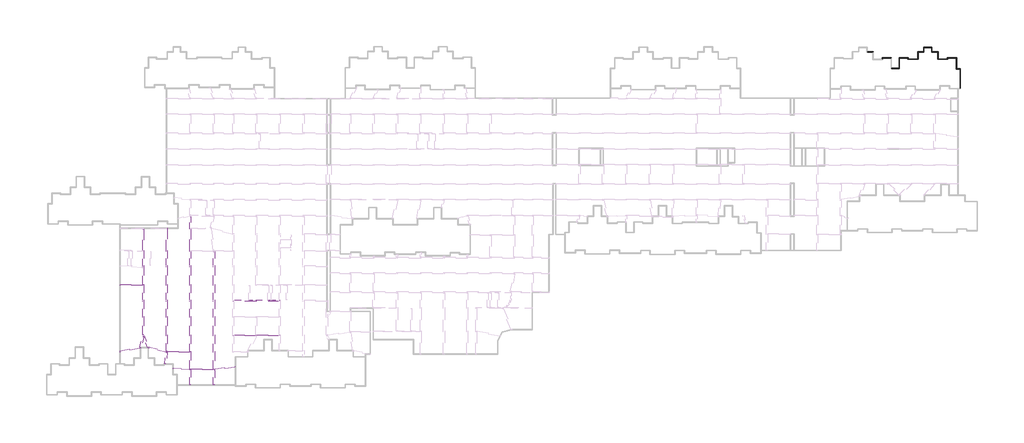
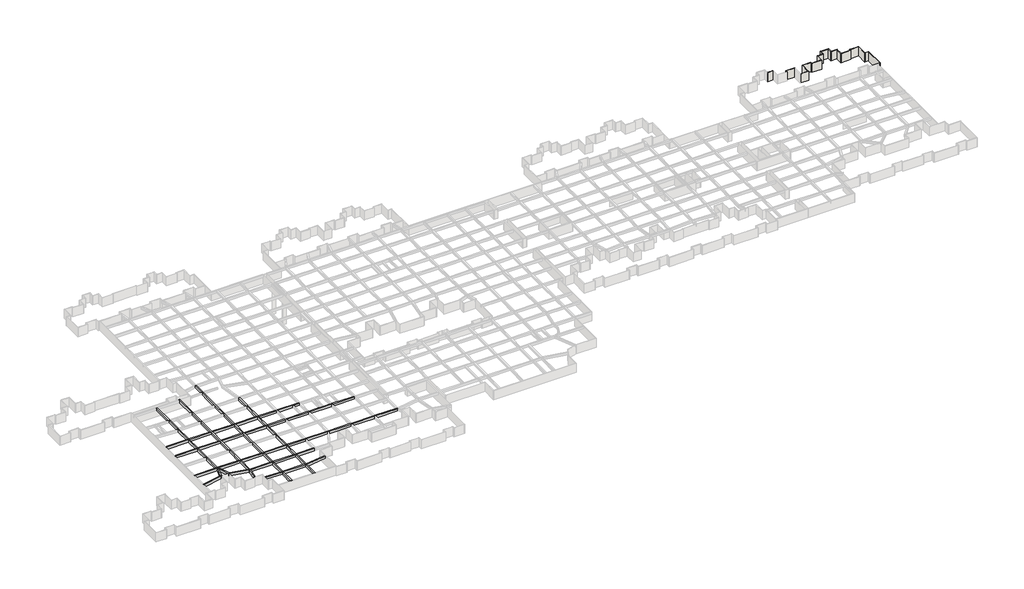
# One storey, part 9 of 16: 21 walls, 16 beams.
"""IFC4 building model written with IfcOpenShell, lengths in millimetres."""

from ifc_helpers import new_model, si_unit, frame, origin, place, context, project, spatial, polyline, outline, extrude, faceted_brep, element, save

model = new_model("IFC4")

# Units and contexts
model_context = context("Model", 3, world=origin())
ifc_project = project(units=[si_unit("LENGTHUNIT", "METRE", prefix="MILLI")], contexts=[model_context])

# Site, building, storey
site = spatial("IfcSite", under=ifc_project)
building = spatial("IfcBuilding", under=site)
storey = spatial("IfcBuildingStorey", under=building, Name="户型图", Elevation=0.0)

# Beams
placement = place(None, origin())
element("IfcBeam", 1, ObjectType="混凝土 - 矩形梁 : KL_beam", at=placement, inside=storey, context=model_context, shape_type="Brep", body=[
    faceted_brep([(208521.0257524, -230392.9293423, 3300.0), (208121.0257524, -230392.9293423, 3300.0), (208121.0257524, -230392.9293423, 2500.0), (208521.0257524, -230392.9293423, 2500.0), (208521.0257524, -225207.0649746, 3300.0), (208521.0257524, -224807.0649746, 3300.0), (208521.0257524, -219234.8916503, 3300.0), (208521.0257524, -218834.8916503, 3300.0), (208521.0257524, -213630.8034485, 3300.0), (208521.0257524, -213230.8034485, 3300.0), (208521.0257524, -207265.1471774, 3300.0), (208521.0257524, -206865.1471774, 3300.0), (208521.0257524, -201765.1471774, 3300.0), (208521.0257524, -201365.1471774, 3300.0), (208521.0257524, -196365.1471774, 3300.0), (208521.0257524, -195965.1471774, 3300.0), (208521.0257524, -189965.1471774, 3300.0), (208521.0257524, -189565.1471774, 3300.0), (208521.0257524, -184765.1471774, 3300.0), (208521.0257524, -184365.1471774, 3300.0), (208521.0257524, -177055.1471774, 3300.0), (208521.0257524, -176755.1471774, 3300.0), (208521.0257524, -172734.8916503, 3300.0), (208320.403704, -172734.8916503, 3300.0), (208121.0257524, -172780.9216773, 3300.0), (208121.0257524, -176755.1471774, 3300.0), (208121.0257524, -177055.1471774, 3300.0), (208121.0257524, -184365.1471774, 3300.0), (208121.0257524, -184765.1471774, 3300.0), (208121.0257524, -189565.1471774, 3300.0), (208121.0257524, -189965.1471774, 3300.0), (208121.0257524, -195965.1471774, 3300.0), (208121.0257524, -196365.1471774, 3300.0), (208121.0257524, -201365.1471774, 3300.0), (208121.0257524, -201765.1471774, 3300.0), (208121.0257524, -206865.1471774, 3300.0), (208121.0257524, -207265.1471774, 3300.0), (208121.0257524, -213230.8034485, 3300.0), (208121.0257524, -213630.8034485, 3300.0), (208121.0257524, -218834.8916503, 3300.0), (208121.0257524, -219234.8916503, 3300.0), (208121.0257524, -224796.3089495, 3300.0), (208121.0257524, -225196.8578879, 3300.0), (208121.0257524, -172780.9216773, 2500.0), (208121.0257524, -184365.1471774, 2500.0), (208121.0257524, -184765.1471774, 2500.0), (208121.0257524, -189565.1471774, 2500.0), (208121.0257524, -189965.1471774, 2500.0), (208121.0257524, -195965.1471774, 2500.0), (208121.0257524, -196365.1471774, 2500.0), (208121.0257524, -201365.1471774, 2500.0), (208121.0257524, -201765.1471774, 2500.0), (208121.0257524, -206865.1471774, 2500.0), (208121.0257524, -207265.1471774, 2500.0), (208121.0257524, -213230.8034485, 2500.0), (208121.0257524, -213630.8034485, 2500.0), (208121.0257524, -218834.8916503, 2500.0), (208121.0257524, -219234.8916503, 2500.0), (208121.0257524, -224796.3089495, 2500.0), (208121.0257524, -225196.8578879, 2500.0), (208320.403704, -172734.8916503, 2500.0), (208521.0257524, -172734.8916503, 2500.0), (208521.0257524, -184365.1471774, 2500.0), (208521.0257524, -184765.1471774, 2500.0), (208521.0257524, -189565.1471774, 2500.0), (208521.0257524, -189965.1471774, 2500.0), (208521.0257524, -195965.1471774, 2500.0), (208521.0257524, -196365.1471774, 2500.0), (208521.0257524, -201365.1471774, 2500.0), (208521.0257524, -201765.1471774, 2500.0), (208521.0257524, -206865.1471774, 2500.0), (208521.0257524, -207265.1471774, 2500.0), (208521.0257524, -213230.8034485, 2500.0), (208521.0257524, -213630.8034485, 2500.0), (208521.0257524, -218834.8916503, 2500.0), (208521.0257524, -219234.8916503, 2500.0), (208521.0257524, -224807.0649746, 2500.0), (208521.0257524, -225207.0649746, 2500.0)], [[[0, 1, 2, 3]], [[1, 0, 4, 5, 6, 7, 8, 9, 10, 11, 12, 13, 14, 15, 16, 17, 18, 19, 20, 21, 22, 23, 24, 25, 26, 27, 28, 29, 30, 31, 32, 33, 34, 35, 36, 37, 38, 39, 40, 41, 42]], [[2, 1, 42, 41, 40, 39, 38, 37, 36, 35, 34, 33, 32, 31, 30, 29, 28, 27, 26, 25, 24, 43, 44, 45, 46, 47, 48, 49, 50, 51, 52, 53, 54, 55, 56, 57, 58, 59]], [[3, 2, 59, 58, 57, 56, 55, 54, 53, 52, 51, 50, 49, 48, 47, 46, 45, 44, 43, 60, 61, 62, 63, 64, 65, 66, 67, 68, 69, 70, 71, 72, 73, 74, 75, 76, 77]], [[0, 3, 77, 76, 75, 74, 73, 72, 71, 70, 69, 68, 67, 66, 65, 64, 63, 62, 61, 22, 21, 20, 19, 18, 17, 16, 15, 14, 13, 12, 11, 10, 9, 8, 7, 6, 5, 4]], [[23, 22, 61, 60]], [[24, 23, 60, 43]]]),
])
element("IfcBeam", 2, ObjectType="混凝土 - 矩形梁 : KL_beam", at=placement, inside=storey, context=model_context, shape_type="Brep", body=[
    faceted_brep([(216206.9772993, -230392.5571059, 3300.0), (216206.9772993, -230392.5571059, 2500.0), (216606.9772993, -230392.5571059, 2500.0), (216606.9772993, -230392.5571059, 3300.0), (216606.9772993, -225295.9807926, 3300.0), (216606.9772993, -224892.0497636, 3300.0), (216606.9772993, -219234.8916503, 3300.0), (216606.9772993, -218834.8916503, 3300.0), (216606.9772993, -213630.8034485, 3300.0), (216606.9772993, -213230.8034485, 3300.0), (216606.9772993, -207265.1471774, 3300.0), (216606.9772993, -206865.1471774, 3300.0), (216606.9772993, -201765.1471774, 3300.0), (216606.9772993, -201365.1471774, 3300.0), (216606.9772993, -196365.1471774, 3300.0), (216606.9772993, -195965.1471774, 3300.0), (216606.9772993, -189965.1471774, 3300.0), (216606.9772993, -189565.1471774, 3300.0), (216606.9772993, -184765.1471774, 3300.0), (216206.9772993, -184765.1471774, 3300.0), (216206.9772993, -189565.1471774, 3300.0), (216206.9772993, -189965.1471774, 3300.0), (216206.9772993, -195965.1471774, 3300.0), (216206.9772993, -196365.1471774, 3300.0), (216206.9772993, -201365.1471774, 3300.0), (216206.9772993, -201765.1471774, 3300.0), (216206.9772993, -206865.1471774, 3300.0), (216206.9772993, -207265.1471774, 3300.0), (216206.9772993, -213230.8034485, 3300.0), (216206.9772993, -213630.8034485, 3300.0), (216206.9772993, -218834.8916503, 3300.0), (216206.9772993, -219234.8916503, 3300.0), (216206.9772993, -224807.0649746, 3300.0), (216206.9772993, -225207.0649746, 3300.0), (216606.9772993, -225295.9807926, 2500.0), (216606.9772993, -224892.0497636, 2500.0), (216606.9772993, -219234.8916503, 2500.0), (216606.9772993, -218834.8916503, 2500.0), (216606.9772993, -213630.8034485, 2500.0), (216606.9772993, -213230.8034485, 2500.0), (216606.9772993, -207265.1471774, 2500.0), (216606.9772993, -206865.1471774, 2500.0), (216606.9772993, -201765.1471774, 2500.0), (216606.9772993, -201365.1471774, 2500.0), (216606.9772993, -196365.1471774, 2500.0), (216606.9772993, -195965.1471774, 2500.0), (216606.9772993, -189965.1471774, 2500.0), (216606.9772993, -189565.1471774, 2500.0), (216606.9772993, -184765.1471774, 2500.0), (216206.9772993, -225207.0649746, 2500.0), (216206.9772993, -224807.0649746, 2500.0), (216206.9772993, -219234.8916503, 2500.0), (216206.9772993, -218834.8916503, 2500.0), (216206.9772993, -213630.8034485, 2500.0), (216206.9772993, -213230.8034485, 2500.0), (216206.9772993, -207265.1471774, 2500.0), (216206.9772993, -206865.1471774, 2500.0), (216206.9772993, -201765.1471774, 2500.0), (216206.9772993, -201365.1471774, 2500.0), (216206.9772993, -196365.1471774, 2500.0), (216206.9772993, -195965.1471774, 2500.0), (216206.9772993, -189965.1471774, 2500.0), (216206.9772993, -189565.1471774, 2500.0), (216206.9772993, -184765.1471774, 2500.0)], [[[0, 1, 2, 3]], [[0, 3, 4, 5, 6, 7, 8, 9, 10, 11, 12, 13, 14, 15, 16, 17, 18, 19, 20, 21, 22, 23, 24, 25, 26, 27, 28, 29, 30, 31, 32, 33]], [[3, 2, 34, 35, 36, 37, 38, 39, 40, 41, 42, 43, 44, 45, 46, 47, 48, 18, 17, 16, 15, 14, 13, 12, 11, 10, 9, 8, 7, 6, 5, 4]], [[2, 1, 49, 50, 51, 52, 53, 54, 55, 56, 57, 58, 59, 60, 61, 62, 63, 48, 47, 46, 45, 44, 43, 42, 41, 40, 39, 38, 37, 36, 35, 34]], [[1, 0, 33, 32, 31, 30, 29, 28, 27, 26, 25, 24, 23, 22, 21, 20, 19, 63, 62, 61, 60, 59, 58, 57, 56, 55, 54, 53, 52, 51, 50, 49]], [[19, 18, 48, 63]]]),
])
element("IfcBeam", 3, ObjectType="混凝土 - 矩形梁 : KL_beam", at=placement, inside=storey, context=model_context, shape_type="SweptSolid", body=[
    extrude(outline(polyline([(223449.910067, -223930.3382806), (223505.5793073, -224326.4455081), (216606.9772993, -225295.9807926), (216606.9772993, -224892.0497636), (223449.910067, -223930.3382806)])), frame((0.0, 0.0, 2500.0), z_axis=(0.0, 0.0, 1.0), x_axis=(1.0, 0.0, 0.0)), (0.0, 0.0, 1.0), 800.0),
])
element("IfcBeam", 4, ObjectType="混凝土 - 矩形梁 : KL_beam", at=placement, inside=storey, context=model_context, shape_type="Brep", body=[
    faceted_brep([(222798.8904026, -219234.8916503, 3300.0), (222798.8904026, -218834.8916503, 3300.0), (216606.9772993, -218834.8916503, 3300.0), (216606.9772993, -219234.8916503, 3300.0), (222798.8904026, -218834.8916503, 2500.0), (216606.9772993, -218834.8916503, 2500.0), (222798.8904026, -219234.8916503, 2500.0), (216606.9772993, -219234.8916503, 2500.0)], [[[0, 1, 2, 3]], [[1, 4, 5, 2]], [[4, 6, 7, 5]], [[6, 0, 3, 7]], [[1, 0, 6, 4]], [[3, 2, 5, 7]]]),
    faceted_brep([(208121.0257524, -218834.8916503, 3300.0), (208121.0257524, -219234.8916503, 3300.0), (208121.0257524, -219234.8916503, 2500.0), (208121.0257524, -218834.8916503, 2500.0), (200545.9052003, -218834.8916503, 3300.0), (200145.9052003, -218834.8916503, 3300.0), (200145.9052003, -219020.9062879, 3300.0), (200145.9052003, -219234.8916503, 3300.0), (200519.7625478, -219234.8916503, 3300.0), (200545.9052003, -218834.8916503, 2500.0), (200145.9052003, -218834.8916503, 2500.0), (200519.7625478, -219234.8916503, 2500.0), (200145.9052003, -219234.8916503, 2500.0), (200145.9052003, -219020.9062879, 2500.0)], [[[0, 1, 2, 3]], [[1, 0, 4, 5, 6, 7, 8]], [[0, 3, 9, 10, 5, 4]], [[3, 2, 11, 12, 13, 10, 9]], [[2, 1, 8, 7, 12, 11]], [[7, 6, 5, 10, 13, 12]]]),
    faceted_brep([(208521.0257524, -219234.8916503, 3300.0), (208521.0257524, -218834.8916503, 3300.0), (208521.0257524, -218834.8916503, 2500.0), (208521.0257524, -219234.8916503, 2500.0), (216206.9772993, -218834.8916503, 3300.0), (216206.9772993, -219234.8916503, 3300.0), (216206.9772993, -219234.8916503, 2500.0), (216206.9772993, -218834.8916503, 2500.0)], [[[0, 1, 2, 3]], [[4, 5, 6, 7]], [[1, 0, 5, 4]], [[2, 1, 4, 7]], [[3, 2, 7, 6]], [[0, 3, 6, 5]]]),
])
element("IfcBeam", 5, ObjectType="混凝土 - 矩形梁 : KL_beam", at=placement, inside=storey, context=model_context, shape_type="Brep", body=[
    faceted_brep([(200545.9052003, -176680.869332, 3300.0), (200145.9052003, -176680.869332, 3300.0), (200145.9052003, -177080.869332, 3300.0), (200145.9052003, -184365.1471774, 3300.0), (200145.9052003, -184765.1471774, 3300.0), (200145.9052003, -189565.1471774, 3300.0), (200145.9052003, -189965.1471774, 3300.0), (200145.9052003, -195965.1471774, 3300.0), (200145.9052003, -196365.1471774, 3300.0), (200145.9052003, -201365.1471774, 3300.0), (200145.9052003, -201765.1471774, 3300.0), (200145.9052003, -206865.1471774, 3300.0), (200145.9052003, -207265.1471774, 3300.0), (200145.9052003, -213230.8034485, 3300.0), (200145.9052003, -213630.8034485, 3300.0), (200145.9052003, -218784.4228576, 3300.0), (200145.9052003, -218834.8916503, 3300.0), (200545.9052003, -218834.8916503, 3300.0), (200545.9052003, -213630.8034485, 3300.0), (200545.9052003, -213230.8034485, 3300.0), (200545.9052003, -207265.1471774, 3300.0), (200545.9052003, -206865.1471774, 3300.0), (200545.9052003, -201765.1471774, 3300.0), (200545.9052003, -201365.1471774, 3300.0), (200545.9052003, -196365.1471774, 3300.0), (200545.9052003, -195965.1471774, 3300.0), (200545.9052003, -189965.1471774, 3300.0), (200545.9052003, -189565.1471774, 3300.0), (200545.9052003, -184765.1471774, 3300.0), (200545.9052003, -184365.1471774, 3300.0), (200145.9052003, -176680.869332, 2500.0), (200145.9052003, -177080.869332, 2500.0), (200145.9052003, -184365.1471774, 2500.0), (200145.9052003, -184765.1471774, 2500.0), (200145.9052003, -189565.1471774, 2500.0), (200145.9052003, -189965.1471774, 2500.0), (200145.9052003, -195965.1471774, 2500.0), (200145.9052003, -196365.1471774, 2500.0), (200145.9052003, -201365.1471774, 2500.0), (200145.9052003, -201765.1471774, 2500.0), (200145.9052003, -206865.1471774, 2500.0), (200145.9052003, -207265.1471774, 2500.0), (200145.9052003, -213230.8034485, 2500.0), (200145.9052003, -213630.8034485, 2500.0), (200145.9052003, -218784.4228576, 2500.0), (200145.9052003, -218834.8916503, 2500.0), (200545.9052003, -176680.869332, 2500.0), (200545.9052003, -184365.1471774, 2500.0), (200545.9052003, -184765.1471774, 2500.0), (200545.9052003, -189565.1471774, 2500.0), (200545.9052003, -189965.1471774, 2500.0), (200545.9052003, -195965.1471774, 2500.0), (200545.9052003, -196365.1471774, 2500.0), (200545.9052003, -201365.1471774, 2500.0), (200545.9052003, -201765.1471774, 2500.0), (200545.9052003, -206865.1471774, 2500.0), (200545.9052003, -207265.1471774, 2500.0), (200545.9052003, -213230.8034485, 2500.0), (200545.9052003, -213630.8034485, 2500.0), (200545.9052003, -218834.8916503, 2500.0)], [[[0, 1, 2, 3, 4, 5, 6, 7, 8, 9, 10, 11, 12, 13, 14, 15, 16, 17, 18, 19, 20, 21, 22, 23, 24, 25, 26, 27, 28, 29]], [[1, 30, 31, 32, 33, 34, 35, 36, 37, 38, 39, 40, 41, 42, 43, 44, 45, 16, 15, 14, 13, 12, 11, 10, 9, 8, 7, 6, 5, 4, 3, 2]], [[30, 46, 47, 48, 49, 50, 51, 52, 53, 54, 55, 56, 57, 58, 59, 45, 44, 43, 42, 41, 40, 39, 38, 37, 36, 35, 34, 33, 32, 31]], [[46, 0, 29, 28, 27, 26, 25, 24, 23, 22, 21, 20, 19, 18, 17, 59, 58, 57, 56, 55, 54, 53, 52, 51, 50, 49, 48, 47]], [[17, 16, 45, 59]], [[1, 0, 46, 30]]]),
])
element("IfcBeam", 6, ObjectType="混凝土 - 矩形梁 : KL_beam", at=placement, inside=storey, context=model_context, shape_type="Brep", body=[
    faceted_brep([(199973.0322053, -223125.0801757, 3300.0), (199576.9249778, -223069.4109354, 3300.0), (199576.9249778, -223069.4109354, 2500.0), (199973.0322053, -223125.0801757, 2500.0), (200519.7625478, -219234.8916503, 3300.0), (200145.9052003, -219234.8916503, 3300.0), (200145.9052003, -219020.9062879, 3300.0), (200122.249653, -219189.2242525, 3300.0), (200145.9052003, -219020.9062879, 2500.0), (200122.249653, -219189.2242525, 2500.0), (200145.9052003, -219234.8916503, 2500.0), (200519.7625478, -219234.8916503, 2500.0)], [[[0, 1, 2, 3]], [[1, 0, 4, 5, 6, 7]], [[2, 1, 7, 6, 8, 9]], [[3, 2, 9, 8, 10, 11]], [[0, 3, 11, 4]], [[10, 5, 4, 11]], [[5, 10, 8, 6]]]),
])
element("IfcBeam", 7, ObjectType="混凝土 - 矩形梁 : KL_beam", at=placement, inside=storey, context=model_context, shape_type="Brep", body=[
    faceted_brep([(193834.6318832, -217762.4339668, 3300.0), (194306.5307519, -217869.5175629, 3300.0), (194129.4851347, -217419.1729302, 3300.0), (192640.1497134, -213630.8034485, 3300.0), (192508.6297316, -213630.8034485, 3300.0), (192210.3490069, -213630.8034485, 3300.0), (192407.3052854, -214131.7941214, 3300.0), (193834.6318832, -217762.4339668, 2500.0), (192210.3490069, -213630.8034485, 2500.0), (192407.3052854, -214131.7941214, 2500.0), (194306.5307519, -217869.5175629, 2500.0), (192508.6297316, -213630.8034485, 2500.0), (192640.1497134, -213630.8034485, 2500.0), (194129.4851347, -217419.1729302, 2500.0)], [[[0, 1, 2, 3, 4, 5, 6]], [[7, 0, 6, 5, 8, 9]], [[10, 7, 9, 8, 11, 12, 13]], [[1, 10, 13, 12, 3, 2]], [[5, 4, 3, 12, 11, 8]], [[1, 0, 7, 10]]]),
])
element("IfcBeam", 8, ObjectType="混凝土 - 矩形梁 : KL_beam", at=placement, inside=storey, context=model_context, shape_type="Brep", body=[
    faceted_brep([(191002.6833489, -217848.9707544, 3300.0), (191439.5808543, -217762.9106202, 3300.0), (192407.3052854, -214131.7941214, 3300.0), (192210.3490069, -213630.8034485, 3300.0), (192126.861975, -213630.8034485, 3300.0), (191117.3552754, -217418.6962767, 3300.0), (191002.6833489, -217848.9707544, 2500.0), (192126.861975, -213630.8034485, 2500.0), (191117.3552754, -217418.6962767, 2500.0), (191439.5808543, -217762.9106202, 2500.0), (192210.3490069, -213630.8034485, 2500.0), (192407.3052854, -214131.7941214, 2500.0)], [[[0, 1, 2, 3, 4, 5]], [[6, 0, 5, 4, 7, 8]], [[9, 6, 8, 7, 10, 11]], [[11, 2, 1, 9]], [[2, 11, 10, 3]], [[4, 3, 10, 7]], [[1, 0, 6, 9]]]),
])
element("IfcBeam", 9, ObjectType="混凝土 - 矩形梁 : KL_beam", at=placement, inside=storey, context=model_context, shape_type="Brep", body=[
    faceted_brep([(192108.6297316, -213230.8034485, 3300.0), (192508.6297316, -213230.8034485, 3300.0), (192508.6297316, -207265.1471774, 3300.0), (192508.6297316, -206865.1471774, 3300.0), (192508.6297316, -201765.1471774, 3300.0), (192508.6297316, -201365.1471774, 3300.0), (192508.6297316, -196365.1471774, 3300.0), (192508.6297316, -195965.1471774, 3300.0), (192508.6297316, -189965.1471774, 3300.0), (192508.6297316, -189565.1471774, 3300.0), (192508.6297316, -184765.1471774, 3300.0), (192508.6297316, -184365.1471774, 3300.0), (192508.6297316, -177080.869332, 3300.0), (192108.6297316, -177080.869332, 3300.0), (192108.6297316, -184358.0411147, 3300.0), (192108.6297316, -184758.2849324, 3300.0), (192108.6297316, -189894.3911524, 3300.0), (192108.6297316, -190294.9400908, 3300.0), (192108.6297316, -195965.1471774, 3300.0), (192108.6297316, -196365.1471774, 3300.0), (192108.6297316, -201365.1471774, 3300.0), (192108.6297316, -201765.1471774, 3300.0), (192108.6297316, -206865.1471774, 3300.0), (192108.6297316, -207265.1471774, 3300.0), (192508.6297316, -213230.8034485, 2500.0), (192508.6297316, -207265.1471774, 2500.0), (192508.6297316, -206865.1471774, 2500.0), (192508.6297316, -201765.1471774, 2500.0), (192508.6297316, -201365.1471774, 2500.0), (192508.6297316, -196365.1471774, 2500.0), (192508.6297316, -195965.1471774, 2500.0), (192508.6297316, -189965.1471774, 2500.0), (192508.6297316, -189565.1471774, 2500.0), (192508.6297316, -184765.1471774, 2500.0), (192508.6297316, -184365.1471774, 2500.0), (192508.6297316, -177080.869332, 2500.0), (192108.6297316, -213230.8034485, 2500.0), (192108.6297316, -207265.1471774, 2500.0), (192108.6297316, -206865.1471774, 2500.0), (192108.6297316, -201765.1471774, 2500.0), (192108.6297316, -201365.1471774, 2500.0), (192108.6297316, -196365.1471774, 2500.0), (192108.6297316, -195965.1471774, 2500.0), (192108.6297316, -190294.9400908, 2500.0), (192108.6297316, -189894.3911524, 2500.0), (192108.6297316, -184758.2849324, 2500.0), (192108.6297316, -184358.0411147, 2500.0), (192108.6297316, -177080.869332, 2500.0)], [[[0, 1, 2, 3, 4, 5, 6, 7, 8, 9, 10, 11, 12, 13, 14, 15, 16, 17, 18, 19, 20, 21, 22, 23]], [[1, 24, 25, 26, 27, 28, 29, 30, 31, 32, 33, 34, 35, 12, 11, 10, 9, 8, 7, 6, 5, 4, 3, 2]], [[24, 36, 37, 38, 39, 40, 41, 42, 43, 44, 45, 46, 47, 35, 34, 33, 32, 31, 30, 29, 28, 27, 26, 25]], [[36, 0, 23, 22, 21, 20, 19, 18, 17, 16, 15, 14, 13, 47, 46, 45, 44, 43, 42, 41, 40, 39, 38, 37]], [[13, 12, 35, 47]], [[24, 1, 0, 36]]]),
])
element("IfcBeam", 10, ObjectType="混凝土 - 矩形梁 : KL_beam", at=placement, inside=storey, context=model_context, shape_type="Brep", body=[
    faceted_brep([(184374.3285911, -195965.1471774, 3300.0), (184374.3285911, -195965.1471774, 2500.0), (184374.3285911, -196365.1471774, 2500.0), (184374.3285911, -196365.1471774, 3300.0), (192108.6297316, -195965.1471774, 3300.0), (192108.6297316, -196365.1471774, 3300.0), (192108.6297316, -196365.1471774, 2500.0), (192108.6297316, -195965.1471774, 2500.0)], [[[0, 1, 2, 3]], [[4, 5, 6, 7]], [[0, 3, 5, 4]], [[3, 2, 6, 5]], [[2, 1, 7, 6]], [[1, 0, 4, 7]]]),
    faceted_brep([(208521.0257524, -195965.1471774, 3300.0), (208521.0257524, -196365.1471774, 3300.0), (216206.9772993, -196365.1471774, 3300.0), (216206.9772993, -195965.1471774, 3300.0), (208521.0257524, -196365.1471774, 2500.0), (216206.9772993, -196365.1471774, 2500.0), (208521.0257524, -195965.1471774, 2500.0), (216206.9772993, -195965.1471774, 2500.0)], [[[0, 1, 2, 3]], [[1, 4, 5, 2]], [[4, 6, 7, 5]], [[6, 0, 3, 7]], [[1, 0, 6, 4]], [[3, 2, 5, 7]]]),
    faceted_brep([(230718.438254, -195965.1471774, 3300.0), (230718.438254, -196365.1471774, 3300.0), (230718.438254, -196365.1471774, 2500.0), (230718.438254, -195965.1471774, 2500.0), (223198.8904026, -195965.1471774, 3300.0), (223198.8904026, -196365.1471774, 3300.0), (228368.438254, -196365.1471774, 3300.0), (228668.438254, -196365.1471774, 3300.0), (223198.8904026, -196365.1471774, 2500.0), (223198.8904026, -195965.1471774, 2500.0)], [[[0, 1, 2, 3]], [[1, 0, 4, 5, 6, 7]], [[2, 1, 7, 6, 5, 8]], [[3, 2, 8, 9]], [[0, 3, 9, 4]], [[5, 4, 9, 8]]]),
    faceted_brep([(208121.0257524, -195965.1471774, 3300.0), (208121.0257524, -196365.1471774, 3300.0), (208121.0257524, -196365.1471774, 2500.0), (208121.0257524, -195965.1471774, 2500.0), (200545.9052003, -195965.1471774, 3300.0), (200545.9052003, -196365.1471774, 3300.0), (200545.9052003, -196365.1471774, 2500.0), (200545.9052003, -195965.1471774, 2500.0)], [[[0, 1, 2, 3]], [[1, 0, 4, 5]], [[2, 1, 5, 6]], [[3, 2, 6, 7]], [[0, 3, 7, 4]], [[5, 4, 7, 6]]]),
    faceted_brep([(216606.9772993, -196365.1471774, 3300.0), (216606.9772993, -195965.1471774, 3300.0), (216606.9772993, -195965.1471774, 2500.0), (216606.9772993, -196365.1471774, 2500.0), (222798.8904026, -195965.1471774, 3300.0), (222798.8904026, -196365.1471774, 3300.0), (222798.8904026, -196365.1471774, 2500.0), (222798.8904026, -195965.1471774, 2500.0)], [[[0, 1, 2, 3]], [[4, 5, 6, 7]], [[1, 0, 5, 4]], [[0, 3, 6, 5]], [[3, 2, 7, 6]], [[2, 1, 4, 7]]]),
    faceted_brep([(200145.9052003, -195965.1471774, 3300.0), (200145.9052003, -196365.1471774, 3300.0), (200145.9052003, -196365.1471774, 2500.0), (200145.9052003, -195965.1471774, 2500.0), (192508.6297316, -195965.1471774, 3300.0), (192508.6297316, -196365.1471774, 3300.0), (192508.6297316, -196365.1471774, 2500.0), (192508.6297316, -195965.1471774, 2500.0)], [[[0, 1, 2, 3]], [[1, 0, 4, 5]], [[2, 1, 5, 6]], [[3, 2, 6, 7]], [[0, 3, 7, 4]], [[5, 4, 7, 6]]]),
])
element("IfcBeam", 11, ObjectType="混凝土 - 矩形梁 : KL_beam", at=placement, inside=storey, context=model_context, shape_type="Brep", body=[
    faceted_brep([(184374.3285911, -201365.1471774, 3300.0), (184374.3285911, -201365.1471774, 2500.0), (184374.3285911, -201765.1471774, 2500.0), (184374.3285911, -201765.1471774, 3300.0), (192108.6297316, -201365.1471774, 3300.0), (192108.6297316, -201765.1471774, 3300.0), (192108.6297316, -201765.1471774, 2500.0), (192108.6297316, -201365.1471774, 2500.0)], [[[0, 1, 2, 3]], [[4, 5, 6, 7]], [[0, 3, 5, 4]], [[3, 2, 6, 5]], [[2, 1, 7, 6]], [[1, 0, 4, 7]]]),
    faceted_brep([(208521.0257524, -201365.1471774, 3300.0), (208521.0257524, -201765.1471774, 3300.0), (216206.9772993, -201765.1471774, 3300.0), (216206.9772993, -201365.1471774, 3300.0), (208521.0257524, -201765.1471774, 2500.0), (216206.9772993, -201765.1471774, 2500.0), (208521.0257524, -201365.1471774, 2500.0), (216206.9772993, -201365.1471774, 2500.0)], [[[0, 1, 2, 3]], [[1, 4, 5, 2]], [[4, 6, 7, 5]], [[6, 0, 3, 7]], [[1, 0, 6, 4]], [[3, 2, 5, 7]]]),
    faceted_brep([(246818.438254, -201365.1471774, 3300.0), (246818.438254, -201765.1471774, 3300.0), (246818.438254, -201765.1471774, 2500.0), (246818.438254, -201365.1471774, 2500.0), (239118.438254, -201765.1471774, 3300.0), (239118.438254, -201365.1471774, 3300.0), (239118.438254, -201365.1471774, 2500.0), (239118.438254, -201765.1471774, 2500.0), (241468.438254, -201365.1471774, 3300.0), (241168.438254, -201365.1471774, 3300.0)], [[[0, 1, 2, 3]], [[4, 5, 6, 7]], [[1, 0, 8, 9, 5, 4]], [[2, 1, 4, 7]], [[3, 2, 7, 6]], [[0, 3, 6, 5, 9, 8]]]),
    faceted_brep([(208121.0257524, -201365.1471774, 3300.0), (208121.0257524, -201765.1471774, 3300.0), (208121.0257524, -201765.1471774, 2500.0), (208121.0257524, -201365.1471774, 2500.0), (200545.9052003, -201365.1471774, 3300.0), (200545.9052003, -201765.1471774, 3300.0), (200545.9052003, -201765.1471774, 2500.0), (200545.9052003, -201365.1471774, 2500.0)], [[[0, 1, 2, 3]], [[1, 0, 4, 5]], [[2, 1, 5, 6]], [[3, 2, 6, 7]], [[0, 3, 7, 4]], [[5, 4, 7, 6]]]),
    faceted_brep([(216606.9772993, -201765.1471774, 3300.0), (216606.9772993, -201365.1471774, 3300.0), (216606.9772993, -201365.1471774, 2500.0), (216606.9772993, -201765.1471774, 2500.0), (222798.8904026, -201365.1471774, 3300.0), (222798.8904026, -201765.1471774, 3300.0), (222798.8904026, -201765.1471774, 2500.0), (222798.8904026, -201365.1471774, 2500.0)], [[[0, 1, 2, 3]], [[4, 5, 6, 7]], [[1, 0, 5, 4]], [[0, 3, 6, 5]], [[3, 2, 7, 6]], [[2, 1, 4, 7]]]),
    faceted_brep([(223198.8904026, -201365.1471774, 3300.0), (223198.8904026, -201765.1471774, 3300.0), (230718.438254, -201765.1471774, 3300.0), (231118.438254, -201765.1471774, 3300.0), (238718.438254, -201765.1471774, 3300.0), (238718.438254, -201365.1471774, 3300.0), (236368.438254, -201365.1471774, 3300.0), (236068.438254, -201365.1471774, 3300.0), (235168.438254, -201365.1471774, 3300.0), (234868.438254, -201365.1471774, 3300.0), (231118.438254, -201365.1471774, 3300.0), (230718.438254, -201365.1471774, 3300.0), (228668.438254, -201365.1471774, 3300.0), (228368.438254, -201365.1471774, 3300.0), (223198.8904026, -201765.1471774, 2500.0), (230718.438254, -201765.1471774, 2500.0), (231118.438254, -201765.1471774, 2500.0), (238718.438254, -201765.1471774, 2500.0), (223198.8904026, -201365.1471774, 2500.0), (230718.438254, -201365.1471774, 2500.0), (231118.438254, -201365.1471774, 2500.0), (238718.438254, -201365.1471774, 2500.0)], [[[0, 1, 2, 3, 4, 5, 6, 7, 8, 9, 10, 11, 12, 13]], [[1, 14, 15, 16, 17, 4, 3, 2]], [[14, 18, 19, 20, 21, 17, 16, 15]], [[18, 0, 13, 12, 11, 10, 9, 8, 7, 6, 5, 21, 20, 19]], [[1, 0, 18, 14]], [[5, 4, 17, 21]]]),
    faceted_brep([(200145.9052003, -201365.1471774, 3300.0), (200145.9052003, -201765.1471774, 3300.0), (200145.9052003, -201765.1471774, 2500.0), (200145.9052003, -201365.1471774, 2500.0), (192508.6297316, -201365.1471774, 3300.0), (192508.6297316, -201765.1471774, 3300.0), (192508.6297316, -201765.1471774, 2500.0), (192508.6297316, -201365.1471774, 2500.0)], [[[0, 1, 2, 3]], [[1, 0, 4, 5]], [[2, 1, 5, 6]], [[3, 2, 6, 7]], [[0, 3, 7, 4]], [[5, 4, 7, 6]]]),
])
element("IfcBeam", 12, ObjectType="混凝土 - 矩形梁 : KL_beam", at=placement, inside=storey, context=model_context, shape_type="Brep", body=[
    faceted_brep([(184374.2189281, -213230.8034485, 3300.0), (184374.2189281, -213230.8034485, 2500.0), (184374.2189281, -213630.8034485, 2500.0), (184374.2189281, -213630.8034485, 3300.0), (192108.6297316, -213372.0637497, 3300.0), (192108.6297316, -213372.0637497, 2500.0), (192108.6297316, -213230.8034485, 2500.0), (192108.6297316, -213230.8034485, 3300.0), (192210.3490069, -213630.8034485, 3300.0), (192210.3490069, -213630.8034485, 2500.0), (192126.861975, -213630.8034485, 3300.0), (192126.861975, -213630.8034485, 2500.0)], [[[0, 1, 2, 3]], [[4, 5, 6, 7]], [[5, 4, 8, 9]], [[0, 3, 10, 8, 4, 7]], [[3, 2, 11, 9, 8, 10]], [[2, 1, 6, 5, 9, 11]], [[1, 0, 7, 6]]]),
    faceted_brep([(254958.4785867, -213230.8034485, 3300.0), (254818.438254, -213230.8034485, 3300.0), (247218.438254, -213230.8034485, 3300.0), (247218.438254, -213630.8034485, 3300.0), (254892.7153783, -213630.8034485, 3300.0), (254989.9592695, -213630.8034485, 3300.0), (247218.438254, -213630.8034485, 2500.0), (254892.7153783, -213630.8034485, 2500.0), (254989.9592695, -213630.8034485, 2500.0), (247218.438254, -213230.8034485, 2500.0), (254818.438254, -213230.8034485, 2500.0), (254958.4785867, -213230.8034485, 2500.0)], [[[0, 1, 2, 3, 4, 5]], [[5, 4, 3, 6, 7, 8]], [[8, 7, 6, 9, 10, 11]], [[2, 1, 0, 11, 10, 9]], [[3, 2, 9, 6]], [[0, 5, 8, 11]]]),
    faceted_brep([(208121.0257524, -213230.8034485, 3300.0), (208121.0257524, -213630.8034485, 3300.0), (208121.0257524, -213630.8034485, 2500.0), (208121.0257524, -213230.8034485, 2500.0), (200545.9052003, -213230.8034485, 3300.0), (200545.9052003, -213630.8034485, 3300.0), (200545.9052003, -213630.8034485, 2500.0), (200545.9052003, -213230.8034485, 2500.0)], [[[0, 1, 2, 3]], [[1, 0, 4, 5]], [[2, 1, 5, 6]], [[3, 2, 6, 7]], [[0, 3, 7, 4]], [[5, 4, 7, 6]]]),
    faceted_brep([(208521.0257524, -213630.8034485, 3300.0), (208521.0257524, -213230.8034485, 3300.0), (208521.0257524, -213230.8034485, 2500.0), (208521.0257524, -213630.8034485, 2500.0), (216206.9772993, -213230.8034485, 3300.0), (216206.9772993, -213630.8034485, 3300.0), (216206.9772993, -213630.8034485, 2500.0), (216206.9772993, -213230.8034485, 2500.0)], [[[0, 1, 2, 3]], [[4, 5, 6, 7]], [[1, 0, 5, 4]], [[0, 3, 6, 5]], [[3, 2, 7, 6]], [[2, 1, 4, 7]]]),
    faceted_brep([(216606.9772993, -213630.8034485, 3300.0), (216606.9772993, -213230.8034485, 3300.0), (216606.9772993, -213230.8034485, 2500.0), (216606.9772993, -213630.8034485, 2500.0), (222798.8904026, -213230.8034485, 3300.0), (222798.8904026, -213630.8034485, 3300.0), (222798.8904026, -213630.8034485, 2500.0), (222798.8904026, -213230.8034485, 2500.0)], [[[0, 1, 2, 3]], [[4, 5, 6, 7]], [[1, 0, 5, 4]], [[0, 3, 6, 5]], [[3, 2, 7, 6]], [[2, 1, 4, 7]]]),
    faceted_brep([(223198.8904026, -213630.8034485, 3300.0), (223198.8904026, -213230.8034485, 3300.0), (223198.8904026, -213230.8034485, 2500.0), (223198.8904026, -213630.8034485, 2500.0), (238718.438254, -213230.8034485, 3300.0), (238718.438254, -213630.8034485, 3300.0), (238718.438254, -213630.8034485, 2500.0), (238718.438254, -213230.8034485, 2500.0), (230585.5823575, -213630.8034485, 3300.0), (231038.6103778, -213630.8034485, 3300.0), (231118.438254, -213230.8034485, 3300.0), (230718.438254, -213230.8034485, 3300.0), (230585.5823575, -213630.8034485, 2500.0), (231038.6103778, -213630.8034485, 2500.0), (230718.438254, -213230.8034485, 2500.0), (231118.438254, -213230.8034485, 2500.0)], [[[0, 1, 2, 3]], [[4, 5, 6, 7]], [[1, 0, 8, 9, 5, 4, 10, 11]], [[0, 3, 12, 13, 6, 5, 9, 8]], [[3, 2, 14, 15, 7, 6, 13, 12]], [[2, 1, 11, 10, 4, 7, 15, 14]]]),
    faceted_brep([(239118.438254, -213630.8034485, 3300.0), (239118.438254, -213230.8034485, 3300.0), (239118.438254, -213230.8034485, 2500.0), (239118.438254, -213630.8034485, 2500.0), (246818.438254, -213230.8034485, 3300.0), (246818.438254, -213630.8034485, 3300.0), (246818.438254, -213630.8034485, 2500.0), (246818.438254, -213230.8034485, 2500.0)], [[[0, 1, 2, 3]], [[4, 5, 6, 7]], [[1, 0, 5, 4]], [[0, 3, 6, 5]], [[3, 2, 7, 6]], [[2, 1, 4, 7]]]),
    faceted_brep([(200145.9052003, -213230.8034485, 3300.0), (200145.9052003, -213630.8034485, 3300.0), (200145.9052003, -213630.8034485, 2500.0), (200145.9052003, -213230.8034485, 2500.0), (192508.6297316, -213230.8034485, 3300.0), (192508.6297316, -213630.8034485, 3300.0), (192640.1497134, -213630.8034485, 3300.0), (192508.6297316, -213630.8034485, 2500.0), (192640.1497134, -213630.8034485, 2500.0), (192508.6297316, -213230.8034485, 2500.0)], [[[0, 1, 2, 3]], [[1, 0, 4, 5, 6]], [[2, 1, 6, 5, 7, 8]], [[3, 2, 8, 7, 9]], [[0, 3, 9, 4]], [[5, 4, 9, 7]]]),
])
element("IfcBeam", 13, ObjectType="混凝土 - 矩形梁 : KL_beam", at=placement, inside=storey, context=model_context, shape_type="SweptSolid", body=[
    extrude(outline(polyline([(184413.3239798, -219146.9437221), (184336.0174411, -218754.4851905), (191117.3552754, -217418.6962767), (191002.6833489, -217848.9707544), (184413.3239798, -219146.9437221)])), frame((0.0, 0.0, 2500.0), z_axis=(0.0, 0.0, 1.0), x_axis=(1.0, 0.0, 0.0)), (0.0, 0.0, 1.0), 800.0),
])
element("IfcBeam", 14, ObjectType="混凝土 - 矩形梁 : KL_beam", at=placement, inside=storey, context=model_context, shape_type="Brep", body=[
    faceted_brep([(200145.9052003, -219020.9062879, 3300.0), (200145.9052003, -218834.8916503, 3300.0), (200145.9052003, -218784.4228576, 3300.0), (194129.4851347, -217419.1729302, 3300.0), (194306.5307519, -217869.5175629, 3300.0), (200122.249653, -219189.2242525, 3300.0), (200145.9052003, -218784.4228576, 2500.0), (194129.4851347, -217419.1729302, 2500.0), (200145.9052003, -218834.8916503, 2500.0), (200145.9052003, -219020.9062879, 2500.0), (200122.249653, -219189.2242525, 2500.0), (194306.5307519, -217869.5175629, 2500.0)], [[[0, 1, 2, 3, 4, 5]], [[2, 6, 7, 3]], [[6, 8, 9, 10, 11, 7]], [[10, 5, 4, 11]], [[6, 2, 1, 0, 9, 8]], [[0, 5, 10, 9]], [[4, 3, 7, 11]]]),
])
element("IfcBeam", 15, ObjectType="混凝土 - 矩形梁 : KL_beam", at=placement, inside=storey, context=model_context, shape_type="SweptSolid", body=[
    extrude(outline(polyline([(202463.299824, -224900.3490362), (202484.2342065, -224500.8972223), (208121.0257524, -224796.3089495), (208121.0257524, -225196.8578879), (202463.299824, -224900.3490362)])), frame((0.0, 0.0, 2500.0), z_axis=(0.0, 0.0, 1.0), x_axis=(1.0, 0.0, 0.0)), (0.0, 0.0, 1.0), 800.0),
])
element("IfcBeam", 16, ObjectType="混凝土 - 矩形梁 : KL_beam", at=placement, inside=storey, context=model_context, shape_type="SweptSolid", body=[
    extrude(outline(polyline([(208521.0257524, -225207.0649746), (208521.0257524, -224807.0649746), (216206.9772993, -224807.0649746), (216206.9772993, -225207.0649746), (208521.0257524, -225207.0649746)])), frame((0.0, 0.0, 2500.0), z_axis=(0.0, 0.0, 1.0), x_axis=(1.0, 0.0, 0.0)), (0.0, 0.0, 1.0), 800.0),
])

# Walls
element("IfcWall", 17, ObjectType="所有墙体", at=placement, inside=storey, context=model_context, shape_type="Brep", body=[
    faceted_brep([(439483.6277241, -116611.319942, 0.0), (441361.840041, -116611.319942, 0.0), (441481.840041, -116611.319942, 0.0), (441481.840041, -116611.319942, 3300.0), (441361.840041, -116611.319942, 3300.0), (439483.6277241, -116611.319942, 3300.0), (439483.6277241, -116491.319942, 0.0), (439483.6277241, -116491.319942, 3300.0), (441481.840041, -116491.319942, 3300.0), (441481.840041, -116491.319942, 0.0)], [[[0, 1, 2, 3, 4, 5]], [[6, 7, 8, 9]], [[2, 1, 0, 6, 9]], [[5, 4, 3, 8, 7]], [[0, 5, 7, 6]], [[3, 2, 9, 8]]]),
])
element("IfcWall", 18, ObjectType="所有墙体", at=placement, inside=storey, context=model_context, shape_type="Brep", body=[
    faceted_brep([(444779.0523526, -118991.319942, 0.0), (444779.0523526, -118598.8141783, 0.0), (444779.0523526, -118478.8141783, 0.0), (444779.0523526, -118478.8141783, 3300.0), (444779.0523526, -118598.8141783, 3300.0), (444779.0523526, -118991.319942, 3300.0), (444659.0523526, -118991.319942, 0.0), (444659.0523526, -118991.319942, 3300.0), (444659.0523526, -118478.8141783, 3300.0), (444659.0523526, -118478.8141783, 0.0)], [[[0, 1, 2, 3, 4, 5]], [[6, 7, 8, 9]], [[2, 1, 0, 6, 9]], [[5, 4, 3, 8, 7]], [[0, 5, 7, 6]], [[3, 2, 9, 8]]]),
])
element("IfcWall", 19, ObjectType="所有墙体", at=placement, inside=storey, context=model_context, shape_type="Brep", body=[
    faceted_brep([(444779.0523526, -118598.8141783, 0.0), (447659.6261242, -118598.8141783, 0.0), (447779.6261242, -118598.8141783, 0.0), (447779.6261242, -118598.8141783, 3300.0), (447659.6261242, -118598.8141783, 3300.0), (444779.0523526, -118598.8141783, 3300.0), (444779.0523526, -118478.8141783, 0.0), (444779.0523526, -118478.8141783, 3300.0), (447779.6261242, -118478.8141783, 3300.0), (447779.6261242, -118478.8141783, 0.0)], [[[0, 1, 2, 3, 4, 5]], [[6, 7, 8, 9]], [[2, 1, 0, 6, 9]], [[5, 4, 3, 8, 7]], [[0, 5, 7, 6]], [[3, 2, 9, 8]]]),
])
element("IfcWall", 20, ObjectType="所有墙体", at=placement, inside=storey, context=model_context, shape_type="Brep", body=[
    faceted_brep([(447779.6261242, -122197.510137, 0.0), (450475.6120305, -122197.510137, 0.0), (450475.6120305, -122197.510137, 3300.0), (447779.6261242, -122197.510137, 3300.0), (447779.6261242, -122077.510137, 0.0), (447779.6261242, -122077.510137, 3300.0), (450355.6120305, -122077.510137, 3300.0), (450475.6120305, -122077.510137, 3300.0), (450475.6120305, -122077.510137, 0.0), (450355.6120305, -122077.510137, 0.0)], [[[0, 1, 2, 3]], [[4, 5, 6, 7, 8, 9]], [[1, 0, 4, 9, 8]], [[3, 2, 7, 6, 5]], [[0, 3, 5, 4]], [[2, 1, 8, 7]]]),
])
element("IfcWall", 21, ObjectType="所有墙体", at=placement, inside=storey, context=model_context, shape_type="Brep", body=[
    faceted_brep([(450475.6120305, -122077.510137, 0.0), (450475.6120305, -118598.8141783, 0.0), (450475.6120305, -118478.8141783, 0.0), (450475.6120305, -118478.8141783, 3300.0), (450475.6120305, -118598.8141783, 3300.0), (450475.6120305, -122077.510137, 3300.0), (450355.6120305, -122077.510137, 0.0), (450355.6120305, -122077.510137, 3300.0), (450355.6120305, -118478.8141783, 3300.0), (450355.6120305, -118478.8141783, 0.0)], [[[0, 1, 2, 3, 4, 5]], [[6, 7, 8, 9]], [[2, 1, 0, 6, 9]], [[5, 4, 3, 8, 7]], [[0, 5, 7, 6]], [[3, 2, 9, 8]]]),
])
element("IfcWall", 22, ObjectType="所有墙体", at=placement, inside=storey, context=model_context, shape_type="Brep", body=[
    faceted_brep([(450475.6120305, -118598.8141783, 0.0), (453359.6296731, -118598.8141783, 0.0), (453479.6296731, -118598.8141783, 0.0), (453479.6296731, -118598.8141783, 3300.0), (453359.6296731, -118598.8141783, 3300.0), (450475.6120305, -118598.8141783, 3300.0), (450475.6120305, -118478.8141783, 0.0), (450475.6120305, -118478.8141783, 3300.0), (453479.6296731, -118478.8141783, 3300.0), (453479.6296731, -118478.8141783, 0.0)], [[[0, 1, 2, 3, 4, 5]], [[6, 7, 8, 9]], [[2, 1, 0, 6, 9]], [[5, 4, 3, 8, 7]], [[0, 5, 7, 6]], [[3, 2, 9, 8]]]),
])
element("IfcWall", 23, ObjectType="所有墙体", at=placement, inside=storey, context=model_context, shape_type="Brep", body=[
    faceted_brep([(453359.6296731, -118598.8141783, 0.0), (453359.6296731, -119026.9395357, 0.0), (453359.6296731, -119026.9395357, 3300.0), (453359.6296731, -118598.8141783, 3300.0), (453479.6296731, -118598.8141783, 0.0), (453479.6296731, -118598.8141783, 3300.0), (453479.6296731, -118906.9395357, 3300.0), (453479.6296731, -119026.9395357, 3300.0), (453479.6296731, -119026.9395357, 0.0), (453479.6296731, -118906.9395357, 0.0)], [[[0, 1, 2, 3]], [[4, 5, 6, 7, 8, 9]], [[1, 0, 4, 9, 8]], [[3, 2, 7, 6, 5]], [[0, 3, 5, 4]], [[2, 1, 8, 7]]]),
])
element("IfcWall", 24, ObjectType="所有墙体", at=placement, inside=storey, context=model_context, shape_type="Brep", body=[
    faceted_brep([(453479.6296731, -119026.9395357, 0.0), (456879.6296731, -119026.9395357, 0.0), (456879.6296731, -119026.9395357, 3300.0), (453479.6296731, -119026.9395357, 3300.0), (453479.6296731, -118906.9395357, 0.0), (453479.6296731, -118906.9395357, 3300.0), (456759.6296731, -118906.9395357, 3300.0), (456879.6296731, -118906.9395357, 3300.0), (456879.6296731, -118906.9395357, 0.0), (456759.6296731, -118906.9395357, 0.0)], [[[0, 1, 2, 3]], [[4, 5, 6, 7, 8, 9]], [[1, 0, 4, 9, 8]], [[3, 2, 7, 6, 5]], [[0, 3, 5, 4]], [[2, 1, 8, 7]]]),
])
element("IfcWall", 25, ObjectType="所有墙体", at=placement, inside=storey, context=model_context, shape_type="Brep", body=[
    faceted_brep([(456879.6296731, -118906.9395357, 0.0), (456879.6296731, -116611.319942, 0.0), (456879.6296731, -116491.319942, 0.0), (456879.6296731, -116491.319942, 3300.0), (456879.6296731, -116611.319942, 3300.0), (456879.6296731, -118906.9395357, 3300.0), (456759.6296731, -118906.9395357, 0.0), (456759.6296731, -118906.9395357, 3300.0), (456759.6296731, -116491.319942, 3300.0), (456759.6296731, -116491.319942, 0.0)], [[[0, 1, 2, 3, 4, 5]], [[6, 7, 8, 9]], [[2, 1, 0, 6, 9]], [[5, 4, 3, 8, 7]], [[0, 5, 7, 6]], [[3, 2, 9, 8]]]),
])
element("IfcWall", 26, ObjectType="所有墙体", at=placement, inside=storey, context=model_context, shape_type="Brep", body=[
    faceted_brep([(456879.6296731, -116611.319942, 0.0), (458881.8508745, -116611.319942, 0.0), (458881.8508745, -116611.319942, 3300.0), (456879.6296731, -116611.319942, 3300.0), (456879.6296731, -116491.319942, 0.0), (456879.6296731, -116491.319942, 3300.0), (458761.8508745, -116491.319942, 3300.0), (458881.8508745, -116491.319942, 3300.0), (458881.8508745, -116491.319942, 0.0), (458761.8508745, -116491.319942, 0.0)], [[[0, 1, 2, 3]], [[4, 5, 6, 7, 8, 9]], [[1, 0, 4, 9, 8]], [[3, 2, 7, 6, 5]], [[0, 3, 5, 4]], [[2, 1, 8, 7]]]),
])
element("IfcWall", 27, ObjectType="所有墙体", at=placement, inside=storey, context=model_context, shape_type="Brep", body=[
    faceted_brep([(458881.8508745, -116491.319942, 0.0), (458881.8508745, -115032.9653688, 0.0), (458881.8508745, -114912.9653688, 0.0), (458881.8508745, -114912.9653688, 3300.0), (458881.8508745, -115032.9653688, 3300.0), (458881.8508745, -116491.319942, 3300.0), (458761.8508745, -116491.319942, 0.0), (458761.8508745, -116491.319942, 3300.0), (458761.8508745, -114912.9653688, 3300.0), (458761.8508745, -114912.9653688, 0.0)], [[[0, 1, 2, 3, 4, 5]], [[6, 7, 8, 9]], [[2, 1, 0, 6, 9]], [[5, 4, 3, 8, 7]], [[0, 5, 7, 6]], [[3, 2, 9, 8]]]),
])
element("IfcWall", 28, ObjectType="所有墙体", at=placement, inside=storey, context=model_context, shape_type="Brep", body=[
    faceted_brep([(458881.8508745, -115032.9653688, 0.0), (461463.613837, -115032.9653688, 0.0), (461583.613837, -115032.9653688, 0.0), (461583.613837, -115032.9653688, 3300.0), (461463.613837, -115032.9653688, 3300.0), (458881.8508745, -115032.9653688, 3300.0), (458881.8508745, -114912.9653688, 0.0), (458881.8508745, -114912.9653688, 3300.0), (461583.613837, -114912.9653688, 3300.0), (461583.613837, -114912.9653688, 0.0)], [[[0, 1, 2, 3, 4, 5]], [[6, 7, 8, 9]], [[2, 1, 0, 6, 9]], [[5, 4, 3, 8, 7]], [[0, 5, 7, 6]], [[3, 2, 9, 8]]]),
])
element("IfcWall", 29, ObjectType="所有墙体", at=placement, inside=storey, context=model_context, shape_type="Brep", body=[
    faceted_brep([(461463.613837, -115032.9653688, 0.0), (461463.613837, -116611.319942, 0.0), (461463.613837, -116611.319942, 3300.0), (461463.613837, -115032.9653688, 3300.0), (461583.613837, -115032.9653688, 0.0), (461583.613837, -115032.9653688, 3300.0), (461583.613837, -116491.319942, 3300.0), (461583.613837, -116611.319942, 3300.0), (461583.613837, -116611.319942, 0.0), (461583.613837, -116491.319942, 0.0)], [[[0, 1, 2, 3]], [[4, 5, 6, 7, 8, 9]], [[1, 0, 4, 9, 8]], [[3, 2, 7, 6, 5]], [[0, 3, 5, 4]], [[2, 1, 8, 7]]]),
])
element("IfcWall", 30, ObjectType="所有墙体", at=placement, inside=storey, context=model_context, shape_type="Brep", body=[
    faceted_brep([(461583.613837, -116611.319942, 0.0), (463561.853863, -116611.319942, 0.0), (463681.853863, -116611.319942, 0.0), (463681.853863, -116611.319942, 3300.0), (463561.853863, -116611.319942, 3300.0), (461583.613837, -116611.319942, 3300.0), (461583.613837, -116491.319942, 0.0), (461583.613837, -116491.319942, 3300.0), (463681.853863, -116491.319942, 3300.0), (463681.853863, -116491.319942, 0.0)], [[[0, 1, 2, 3, 4, 5]], [[6, 7, 8, 9]], [[2, 1, 0, 6, 9]], [[5, 4, 3, 8, 7]], [[0, 5, 7, 6]], [[3, 2, 9, 8]]]),
])
element("IfcWall", 31, ObjectType="所有墙体", at=placement, inside=storey, context=model_context, shape_type="Brep", body=[
    faceted_brep([(463561.853863, -116611.319942, 0.0), (463561.853863, -119026.9395357, 0.0), (463561.853863, -119026.9395357, 3300.0), (463561.853863, -116611.319942, 3300.0), (463681.853863, -116611.319942, 0.0), (463681.853863, -116611.319942, 3300.0), (463681.853863, -118906.9395357, 3300.0), (463681.853863, -119026.9395357, 3300.0), (463681.853863, -119026.9395357, 0.0), (463681.853863, -118906.9395357, 0.0)], [[[0, 1, 2, 3]], [[4, 5, 6, 7, 8, 9]], [[1, 0, 4, 9, 8]], [[3, 2, 7, 6, 5]], [[0, 3, 5, 4]], [[2, 1, 8, 7]]]),
])
element("IfcWall", 32, ObjectType="所有墙体", at=placement, inside=storey, context=model_context, shape_type="Brep", body=[
    faceted_brep([(463681.853863, -119026.9395357, 0.0), (466979.1603345, -119026.9395357, 0.0), (466979.1603345, -119026.9395357, 3300.0), (463681.853863, -119026.9395357, 3300.0), (463681.853863, -118906.9395357, 0.0), (463681.853863, -118906.9395357, 3300.0), (466859.1603345, -118906.9395357, 3300.0), (466979.1603345, -118906.9395357, 3300.0), (466979.1603345, -118906.9395357, 0.0), (466859.1603345, -118906.9395357, 0.0)], [[[0, 1, 2, 3]], [[4, 5, 6, 7, 8, 9]], [[1, 0, 4, 9, 8]], [[3, 2, 7, 6, 5]], [[0, 3, 5, 4]], [[2, 1, 8, 7]]]),
])
element("IfcWall", 33, ObjectType="所有墙体", at=placement, inside=storey, context=model_context, shape_type="Brep", body=[
    faceted_brep([(466979.1603345, -118906.9395357, 0.0), (466979.1603345, -118598.8141783, 0.0), (466979.1603345, -118478.8141783, 0.0), (466979.1603345, -118478.8141783, 3300.0), (466979.1603345, -118598.8141783, 3300.0), (466979.1603345, -118906.9395357, 3300.0), (466859.1603345, -118906.9395357, 0.0), (466859.1603345, -118906.9395357, 3300.0), (466859.1603345, -118478.8141783, 3300.0), (466859.1603345, -118478.8141783, 0.0)], [[[0, 1, 2, 3, 4, 5]], [[6, 7, 8, 9]], [[2, 1, 0, 6, 9]], [[5, 4, 3, 8, 7]], [[0, 5, 7, 6]], [[3, 2, 9, 8]]]),
])
element("IfcWall", 34, ObjectType="所有墙体", at=placement, inside=storey, context=model_context, shape_type="Brep", body=[
    faceted_brep([(466979.1603345, -118598.8141783, 0.0), (469959.6400085, -118598.8141783, 0.0), (470079.6400085, -118598.8141783, 0.0), (470079.6400085, -118598.8141783, 3300.0), (469959.6400085, -118598.8141783, 3300.0), (466979.1603345, -118598.8141783, 3300.0), (466979.1603345, -118478.8141783, 0.0), (466979.1603345, -118478.8141783, 3300.0), (470079.6400085, -118478.8141783, 3300.0), (470079.6400085, -118478.8141783, 0.0)], [[[0, 1, 2, 3, 4, 5]], [[6, 7, 8, 9]], [[2, 1, 0, 6, 9]], [[5, 4, 3, 8, 7]], [[0, 5, 7, 6]], [[3, 2, 9, 8]]]),
])
element("IfcWall", 35, ObjectType="所有墙体", at=placement, inside=storey, context=model_context, shape_type="Brep", body=[
    faceted_brep([(469959.6400085, -118598.8141783, 0.0), (469959.6400085, -122345.4654954, 0.0), (469959.6400085, -122345.4654954, 3300.0), (469959.6400085, -118598.8141783, 3300.0), (470079.6400085, -118598.8141783, 0.0), (470079.6400085, -118598.8141783, 3300.0), (470079.6400085, -122225.4654954, 3300.0), (470079.6400085, -122345.4654954, 3300.0), (470079.6400085, -122345.4654954, 0.0), (470079.6400085, -122225.4654954, 0.0)], [[[0, 1, 2, 3]], [[4, 5, 6, 7, 8, 9]], [[1, 0, 4, 9, 8]], [[3, 2, 7, 6, 5]], [[0, 3, 5, 4]], [[2, 1, 8, 7]]]),
])
element("IfcWall", 36, ObjectType="所有墙体", at=placement, inside=storey, context=model_context, shape_type="Brep", body=[
    faceted_brep([(470079.6400085, -122345.4654954, 0.0), (471205.459909, -122345.4654954, 0.0), (471325.459909, -122345.4654954, 0.0), (471325.459909, -122345.4654954, 3300.0), (471205.459909, -122345.4654954, 3300.0), (470079.6400085, -122345.4654954, 3300.0), (470079.6400085, -122225.4654954, 0.0), (470079.6400085, -122225.4654954, 3300.0), (471325.459909, -122225.4654954, 3300.0), (471325.459909, -122225.4654954, 0.0)], [[[0, 1, 2, 3, 4, 5]], [[6, 7, 8, 9]], [[2, 1, 0, 6, 9]], [[5, 4, 3, 8, 7]], [[0, 5, 7, 6]], [[3, 2, 9, 8]]]),
])
element("IfcWall", 37, ObjectType="所有墙体", at=placement, inside=storey, context=model_context, shape_type="Brep", body=[
    faceted_brep([(471205.459909, -122345.4654954, 0.0), (471205.459909, -129026.8599361, 0.0), (471205.459909, -129146.8599361, 0.0), (471205.459909, -129146.8599361, 3300.0), (471205.459909, -129026.8599361, 3300.0), (471205.459909, -122345.4654954, 3300.0), (471325.459909, -122345.4654954, 0.0), (471325.459909, -122345.4654954, 3300.0), (471325.459909, -129146.8599361, 3300.0), (471325.459909, -129146.8599361, 0.0)], [[[0, 1, 2, 3, 4, 5]], [[6, 7, 8, 9]], [[2, 1, 0, 6, 9]], [[5, 4, 3, 8, 7]], [[0, 5, 7, 6]], [[3, 2, 9, 8]]]),
])

save(model, "model.ifc")

# Revit data of these elements
# Type "混凝土 - 矩形梁 : KL_beam"
#   Length [instance default] = 1524 mm
#   b = 400 mm
#   h = 800 mm
#   Structural Material [instance default] = 混凝土 - 现场浇注混凝土
#   Assembly Code = ""
# Type "所有墙体"
#   Layers, outside or top first: 120 mm "默认" (function 1)
# Elements 1, 2, 3, 4, 5, 6, 7, 8, 9, 10, 11, 12, 13, 14, 15, 16 (IfcBeam, "混凝土 - 矩形梁 : KL_beam")
#   Comments = ""
#   Structural Material = none
#   Phase Created = 新构造
# Elements 17, 18, 19, 20, 21, 22, 23, 24, 25, 26, 27, 28, 29, 30, 31, 32, 33, 34, 35, 36, 37 (IfcWall, "所有墙体")
#   Top Offset = 0 mm
#   Base Offset = 0 mm
#   wall height = 3300 mm
#   Phase Created = 新构造
#   Base Constraint = 户型图
#   Top Constraint = 层高
#   Materials on its faces: "默认"
# Materials
#   "混凝土 - 现场浇注混凝土": class "混凝土", colour RGB 192 192 192, transparency 0
#   "默认": class "其他", colour RGB 192 192 192, transparency 0, Cost = 0
